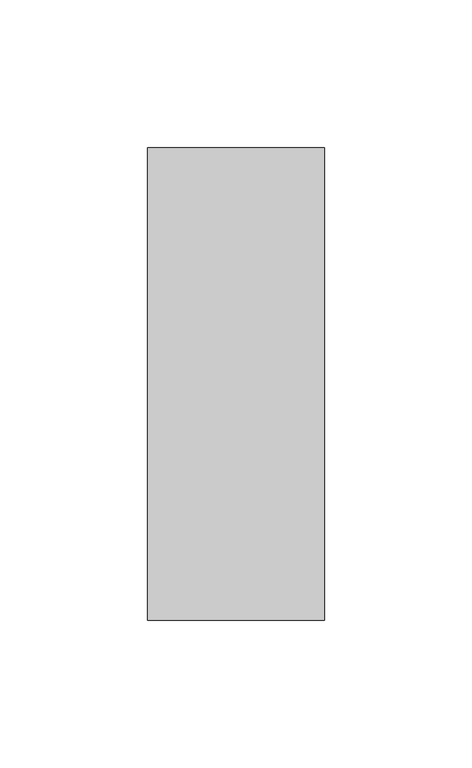
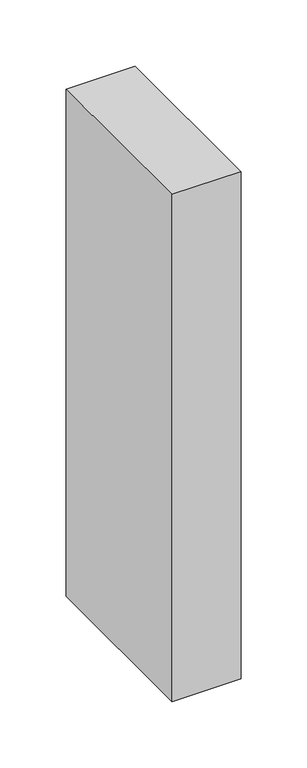
"""IFC4 building model written with IfcOpenShell, lengths in millimetres: column geometry, Madeira de lei-Coluna : Pontalete 6X16cm."""

from ifc_helpers import new_model, si_unit, frame, origin, place, context, project, spatial, polyline, outline, extrude, source, transform, mapped, element, save


def column_6c15bf79(model_context):
    return source(origin(), model_context, "Body", "SweptSolid", [
        extrude(outline(polyline([(30.0, 80.0), (30.0, -80.0), (-30.0, -80.0), (-30.0, 80.0), (30.0, 80.0)])), frame((0.0, 0.0, 6710.0), z_axis=(0.0, 0.0, 1.0), x_axis=(1.0, 0.0, 0.0)), (0.0, 0.0, 1.0), 467.5),
    ])


if __name__ == "__main__":
    model = new_model("IFC4")
    model_context = context("Model", 3, world=origin())
    ifc_project = project(units=[si_unit("LENGTHUNIT", "METRE", prefix="MILLI")], contexts=[model_context])
    site = spatial("IfcSite", under=ifc_project)
    building = spatial("IfcBuilding", under=site)
    placement = place(None, origin())
    column_shape = column_6c15bf79(model_context)
    element("IfcColumn", 1, ObjectType="Madeira de lei-Coluna : Pontalete 6X16cm", at=placement, inside=building, context=model_context, shape_type="MappedRepresentation", body=[
        mapped(column_shape, transform((0.0, 0.0, 0.0), x_axis=(1.0, 0.0, 0.0), y_axis=(0.0, 1.0, 0.0), z_axis=(0.0, 0.0, 1.0))),
    ])
    save(model, "model.ifc")

# Revit data of these elements
# Type "Madeira de lei-Coluna : Pontalete 6X16cm"
#   A = 0.01952 m²
#   b = 0.06 m
#   d = 0.16 m
#   Structural Material [instance default] = none
#   Assembly Code = ""
# Element 1 (IfcColumn, "Madeira de lei-Coluna : Pontalete 6X16cm")
#   Structural Material = .MADEIRAMENTO
#   Materials on its faces: ".MADEIRAMENTO"
# Materials
#   ".MADEIRAMENTO": class ".CC_MADEIRAS", colour RGB 212 179 113, transparency 0, Cost = 0
